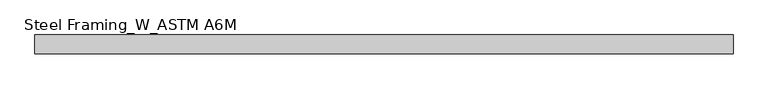
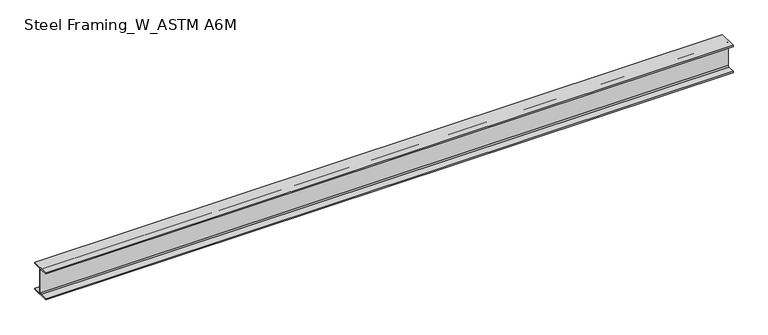
"""IFC4 building model written with IfcOpenShell, lengths in millimetres: beam geometry, Steel Framing_W_ASTM A6M : H_SB_AR_S02_W200x31.3_RB4."""

import ifcopenshell
import ifcopenshell.guid

model = None  # the IFC model being written
_history = None  # IfcOwnerHistory: only IFC2X3 demands one
_inside = {}  # id of a spatial element -> (the spatial element, [elements in it])
_under = {}  # id of a project, library or spatial element -> (it, [spatial elements below it])
_declared = {}  # id of a project -> (the project, [libraries it declares])
_typed = {}  # id of a type object -> (the type object, [elements of that type])
_made_of = {}  # id of a material, layer set ... -> (it, [elements and type objects made of it])


def new_model(schema):
    """Start an empty IFC model of exactly this schema.

    Asked for "IFC4X3", IfcOpenShell would pick the latest addendum, in which some entities
    have other attributes; the version numbers below select the first issue.
    IFC2X3 requires an IfcOwnerHistory on every rooted entity: one is made here for all.
    """
    global model, _history
    if schema == "IFC4X3":
        model = ifcopenshell.file(schema_version=(4, 3, 0, 0))
    else:
        model = ifcopenshell.file(schema=schema)
    _inside.clear()
    _under.clear()
    _declared.clear()
    _typed.clear()
    _made_of.clear()
    _history = None
    if model.schema == "IFC2X3":
        org = make("IfcOrganization", Name="unknown")
        user = make(
            "IfcPersonAndOrganization",
            ThePerson=make("IfcPerson", FamilyName="unknown"),
            TheOrganization=org,
        )
        app = make(
            "IfcApplication",
            ApplicationDeveloper=org,
            Version="unknown",
            ApplicationFullName="unknown",
            ApplicationIdentifier="unknown",
        )
        _history = make(
            "IfcOwnerHistory",
            OwningUser=user,
            OwningApplication=app,
            ChangeAction="ADDED",
            CreationDate=0,
        )
    return model


def make(cls, **values):
    """One entity of the class cls with the attributes given. An attribute that is None is left unset."""
    return model.create_entity(
        cls, **{name: value for name, value in values.items() if value is not None}
    )


def rooted(cls, **values):
    """An entity with a GlobalId (a new one), such as an element, a storey or a relation."""
    return make(cls, GlobalId=ifcopenshell.guid.new(), OwnerHistory=_history, **values)


def si_unit(unit_type, name, prefix=None):
    """IfcSIUnit, for example si_unit("LENGTHUNIT", "METRE", prefix="MILLI")."""
    return make("IfcSIUnit", UnitType=unit_type, Prefix=prefix, Name=name)


def assignment(units):
    """IfcUnitAssignment: the units of a project."""
    return None if units is None else make("IfcUnitAssignment", Units=units)


def point(xyz):
    """IfcCartesianPoint."""
    return None if xyz is None else make("IfcCartesianPoint", Coordinates=xyz)


def direction(xyz):
    """IfcDirection."""
    return None if xyz is None else make("IfcDirection", DirectionRatios=xyz)


def frame(location, z_axis=None, x_axis=None):
    """IfcAxis2Placement3D, a coordinate frame: its origin and axes. An axis left out is left unset."""
    return make(
        "IfcAxis2Placement3D",
        Location=point(location),
        Axis=direction(z_axis),
        RefDirection=direction(x_axis),
    )


def frame_2d(location, x_axis=None):
    """IfcAxis2Placement2D, a coordinate frame in the plane: its origin and x axis."""
    return make(
        "IfcAxis2Placement2D", Location=point(location), RefDirection=direction(x_axis)
    )


def origin():
    """The frame at (0, 0, 0) with its axes left unset."""
    return frame((0.0, 0.0, 0.0))


def place(relative_to, where):
    """IfcLocalPlacement: puts the frame where relative to a parent placement (None: the world)."""
    return make(
        "IfcLocalPlacement", PlacementRelTo=relative_to, RelativePlacement=where
    )


def context(
    kind, dimensions, precision=None, world=None, true_north=None, identifier=None
):
    """IfcGeometricRepresentationContext, for example the 3D "Model" context."""
    return make(
        "IfcGeometricRepresentationContext",
        ContextIdentifier=identifier,
        ContextType=kind,
        CoordinateSpaceDimension=dimensions,
        Precision=precision,
        WorldCoordinateSystem=world,
        TrueNorth=true_north,
    )


def project(units=None, contexts=None):
    """IfcProject with its units and contexts."""
    return rooted(
        "IfcProject",
        Name="project",
        RepresentationContexts=contexts,
        UnitsInContext=assignment(units),
    )


def spatial(cls, under=None, at=None, **own):
    """A site, building, storey or space (cls), placed at a placement, below another one or the project."""
    s = rooted(cls, ObjectPlacement=at, **own)
    if under is not None:
        _under.setdefault(under.id(), (under, []))[1].append(s)
    return s


def polyline(points):
    """IfcPolyline through the points."""
    return make("IfcPolyline", Points=[point(p) for p in points])


def circle_curve(where, radius):
    """IfcCircle in the frame where."""
    return make("IfcCircle", Position=where, Radius=radius)


def trimmed(basis, trim1, trim2, sense, master):
    """IfcTrimmedCurve: the piece of a basis curve between two trims."""
    return make(
        "IfcTrimmedCurve",
        BasisCurve=basis,
        Trim1=trim1,
        Trim2=trim2,
        SenseAgreement=sense,
        MasterRepresentation=master,
    )


def segment(curve, same_sense, transition):
    """IfcCompositeCurveSegment."""
    return make(
        "IfcCompositeCurveSegment",
        Transition=transition,
        SameSense=same_sense,
        ParentCurve=curve,
    )


def composite_curve(segments, self_intersect=None):
    """IfcCompositeCurve: segments joined end to end."""
    return make("IfcCompositeCurve", Segments=segments, SelfIntersect=self_intersect)


def outline(outer, holes=None, kind="AREA"):
    """IfcArbitraryClosedProfileDef: a profile drawn as a closed curve; with holes, ...WithVoids."""
    if holes is None:
        return make("IfcArbitraryClosedProfileDef", ProfileType=kind, OuterCurve=outer)
    return make(
        "IfcArbitraryProfileDefWithVoids",
        ProfileType=kind,
        OuterCurve=outer,
        InnerCurves=holes,
    )


def extrude(swept, where, along, depth):
    """IfcExtrudedAreaSolid: the profile swept, set in the frame where, extruded along a direction by depth."""
    return make(
        "IfcExtrudedAreaSolid",
        SweptArea=swept,
        Position=where,
        ExtrudedDirection=direction(along),
        Depth=depth,
    )


def shape(context_of_items, identifier, shape_type, items):
    """IfcShapeRepresentation: the items that make up one representation, for example the "Body"."""
    return make(
        "IfcShapeRepresentation",
        ContextOfItems=context_of_items,
        RepresentationIdentifier=identifier,
        RepresentationType=shape_type,
        Items=items,
    )


def source(mapping_origin, context_of_items, identifier, shape_type, items):
    """IfcRepresentationMap: a shape defined once, which mapped items show again and again."""
    return make(
        "IfcRepresentationMap",
        MappingOrigin=mapping_origin,
        MappedRepresentation=shape(context_of_items, identifier, shape_type, items),
    )


def transform(
    local_origin,
    x_axis=None,
    y_axis=None,
    z_axis=None,
    scale=None,
    scale2=None,
    scale3=None,
    uniform=True,
):
    """IfcCartesianTransformationOperator3D, or its non-uniform kind. x_axis, y_axis, z_axis: its Axis1, 2, 3."""
    if uniform:
        return make(
            "IfcCartesianTransformationOperator3D",
            Axis1=direction(x_axis),
            Axis2=direction(y_axis),
            LocalOrigin=point(local_origin),
            Scale=scale,
            Axis3=direction(z_axis),
        )
    return make(
        "IfcCartesianTransformationOperator3DnonUniform",
        Axis1=direction(x_axis),
        Axis2=direction(y_axis),
        LocalOrigin=point(local_origin),
        Scale=scale,
        Axis3=direction(z_axis),
        Scale2=scale2,
        Scale3=scale3,
    )


def mapped(mapping_source, mapping_target):
    """IfcMappedItem: shows the shape of a source again, moved by a transform."""
    return make(
        "IfcMappedItem", MappingSource=mapping_source, MappingTarget=mapping_target
    )


def made_of(thing, what):
    """Note that an element or type object is made of a material, layer set ...; save() writes the relation."""
    if what is not None:
        _made_of.setdefault(what.id(), (what, []))[1].append(thing)
    return thing


def element(
    cls,
    number,
    at=None,
    inside=None,
    cuts=None,
    type_object=None,
    material=None,
    context=None,
    identifier="Body",
    shape_type=None,
    held_by="IfcProductDefinitionShape",
    body=None,
    shapes=None,
    **own,
):
    """One element of the class cls, such as IfcWall. Its Tag is "e" and its number.

    at: its placement. inside: the storey or other place that contains it. cuts: it is an
    opening in that element (IfcRelVoidsElement). A single representation is given by context,
    identifier, shape_type and body (its items); several are given by shapes. held_by: the class
    of the entity that holds the representations. save() writes the other relations.
    """
    e = rooted(cls, Tag="e%d" % number, ObjectPlacement=at, **own)
    if body is not None:
        shapes = [shape(context, identifier, shape_type, body)]
    if shapes is not None:
        e.Representation = make(held_by, Representations=shapes)
    if inside is not None:
        _inside.setdefault(inside.id(), (inside, []))[1].append(e)
    if cuts is not None:
        rooted(
            "IfcRelVoidsElement", RelatingBuildingElement=cuts, RelatedOpeningElement=e
        )
    if type_object is not None:
        _typed.setdefault(type_object.id(), (type_object, []))[1].append(e)
    return made_of(e, material)


def aggregate(whole, parts):
    """IfcRelAggregates: a whole, such as a stair, and the parts it consists of."""
    return rooted("IfcRelAggregates", RelatingObject=whole, RelatedObjects=parts)


def save(model, path):
    """Write the relations noted so far, then the file.

    IfcRelAggregates (storeys below a building ...), IfcRelContainedInSpatialStructure (elements
    in a storey), IfcRelDefinesByType, IfcRelAssociatesMaterial and IfcRelDeclares: one each for
    every whole, place, type object, material and project.
    """
    for whole, parts in _under.values():
        aggregate(whole, parts)
    for where, things in _inside.values():
        rooted(
            "IfcRelContainedInSpatialStructure",
            RelatedElements=things,
            RelatingStructure=where,
        )
    for kind, things in _typed.values():
        rooted("IfcRelDefinesByType", RelatedObjects=things, RelatingType=kind)
    for what, things in _made_of.values():
        rooted("IfcRelAssociatesMaterial", RelatedObjects=things, RelatingMaterial=what)
    for by, libraries in _declared.values():
        rooted("IfcRelDeclares", RelatingContext=by, RelatedDefinitions=libraries)
    model.write(path)


def steel_framing_w_astm_a6m_565b4d53(model_context):
    return source(origin(), model_context, "Body", "SweptSolid", [
        extrude(outline(composite_curve([segment(polyline([(67.0, -94.8), (67.0, -105.0), (-67.0, -105.0), (-67.0, -94.8), (-10.775, -94.8)]), True, "CONTINUOUS"), segment(trimmed(circle_curve(frame_2d((-10.775, -87.2)), 7.6), [point((-10.775, -94.8))], [point((-3.175, -87.2))], True, "CARTESIAN"), True, "CONTINUOUS"), segment(polyline([(-3.175, -87.2), (-3.175, 87.2)]), True, "CONTINUOUS"), segment(trimmed(circle_curve(frame_2d((-10.775, 87.2)), 7.6), [point((-3.175, 87.2))], [point((-10.775, 94.8))], True, "CARTESIAN"), True, "CONTINUOUS"), segment(polyline([(-10.775, 94.8), (-67.0, 94.8), (-67.0, 105.0), (67.0, 105.0), (67.0, 94.8), (10.775, 94.8)]), True, "CONTINUOUS"), segment(trimmed(circle_curve(frame_2d((10.775, 87.2)), 7.6), [point((10.775, 94.8))], [point((3.175, 87.2))], True, "CARTESIAN"), True, "CONTINUOUS"), segment(polyline([(3.175, 87.2), (3.175, -87.2)]), True, "CONTINUOUS"), segment(trimmed(circle_curve(frame_2d((10.775, -87.2)), 7.6), [point((3.175, -87.2))], [point((10.775, -94.8))], True, "CARTESIAN"), True, "CONTINUOUS"), segment(polyline([(10.775, -94.8), (67.0, -94.8)]), True, "CONTINUOUS")], self_intersect=False)), frame((-2500.0, 0.0, 0.0), z_axis=(1.0, 0.0, 0.0), x_axis=(0.0, 1.0, 0.0)), (0.0, 0.0, 1.0), 5000.0),
    ])


if __name__ == "__main__":
    model = new_model("IFC4")
    model_context = context("Model", 3, world=origin())
    ifc_project = project(units=[si_unit("LENGTHUNIT", "METRE", prefix="MILLI")], contexts=[model_context])
    site = spatial("IfcSite", under=ifc_project)
    building = spatial("IfcBuilding", under=site)
    placement = place(None, origin())
    steel_framing_w_astm_a6m_shape = steel_framing_w_astm_a6m_565b4d53(model_context)
    element("IfcBeam", 1, ObjectType="Steel Framing_W_ASTM A6M : H_SB_AR_S02_W200x31.3_RB4", at=placement, inside=building, context=model_context, shape_type="MappedRepresentation", body=[
        mapped(steel_framing_w_astm_a6m_shape, transform((0.0, 0.0, 0.0), x_axis=(1.0, 0.0, 0.0), y_axis=(0.0, 1.0, 0.0), z_axis=(0.0, 0.0, 1.0))),
    ])
    save(model, "model.ifc")

# Revit data of these elements
# Type "Steel Framing_W_ASTM A6M : H_SB_AR_S02_W200x31.3_RB4"
#   Section Name Key = "W8x21"
#   Width = 13.4 cm
#   Web Thickness = 0.635 cm
#   Web Fillet = 0.76 cm
#   Warping Constant = 40800.0 cm⁶
#   Torsional Moment of Inertia = 11.70 cm⁴
#   Section Area = 39.7 cm²
#   Plastic Modulus weak axis = 93.2 cm³
#   Plastic Modulus strong axis = 334.0 cm³
#   Perimeter = 0.93 m²/m
#   Nominal Weight = 31.30 kgf/m
#   Moment of Inertia weak axis = 407.00 cm⁴
#   Moment of Inertia strong axis = 3130.00 cm⁴
#   Height = 21.0 cm
#   Flange Thickness = 1.02 cm
#   Elastic Modulus weak axis = 60.8 cm³
#   Elastic Modulus strong axis = 298.0 cm³
#   Centroid Vertical = 10.5 cm
#   Centroid Horizontal = 6.7 cm
#   Length [instance default] = 1500 mm
#   Structural Material [instance default] = Steel, 45-345
#   Bolt Spacing = 0
#   Assembly Code = ""
# Element 1 (IfcBeam, "Steel Framing_W_ASTM A6M : H_SB_AR_S02_W200x31.3_RB4")
#   Materials on its faces: "Steel, 45-345"
# Materials
#   "Steel, 45-345": class "Metal", colour RGB 189 187 185, transparency 0, Description = "Steel 345 MPa", Cost = 0
